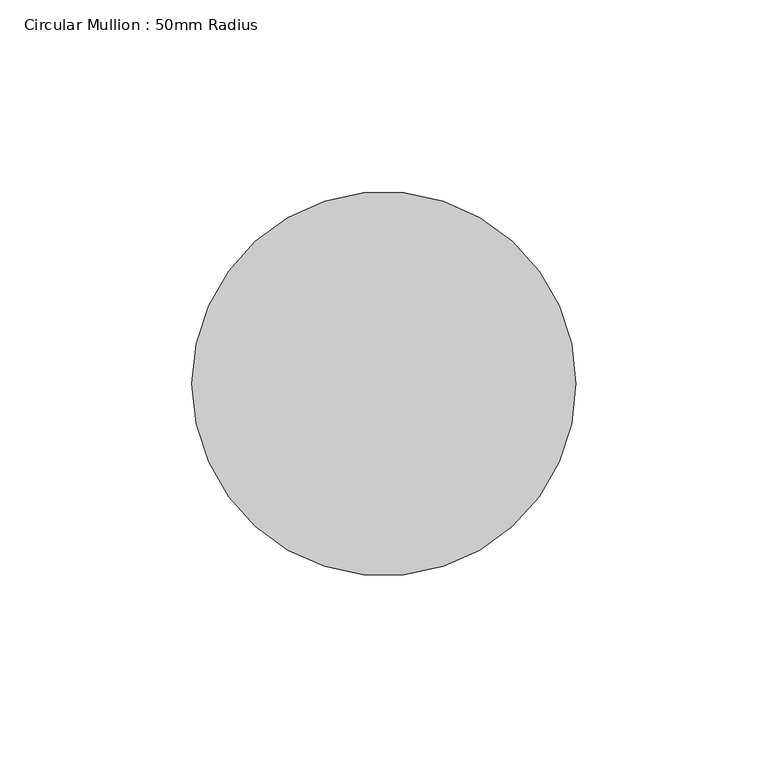
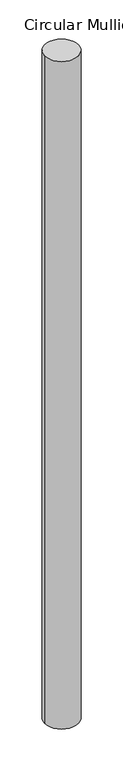
"""IFC4 building model written with IfcOpenShell, lengths in millimetres: member geometry, Circular Mullion : 50mm Radius."""

from ifc_helpers import new_model, si_unit, point, frame, frame_2d, origin, place, context, project, spatial, circle_curve, trimmed, segment, composite_curve, outline, extrude, source, transform, mapped, element, save


def circular_mullion_50mm_radius_f1cf2dd3(model_context):
    return source(origin(), model_context, "Body", "SweptSolid", [
        extrude(outline(composite_curve([segment(trimmed(circle_curve(frame_2d((-50.0, 0.0)), 50.0), [point((0.0, 0.0))], [point((-100.0, 0.0))], False, "CARTESIAN"), True, "CONTINUOUS"), segment(trimmed(circle_curve(frame_2d((-50.0, 0.0)), 50.0), [point((-100.0, 0.0))], [point((0.0, 0.0))], False, "CARTESIAN"), True, "CONTINUOUS")], self_intersect=False)), frame((0.0, 0.0, -2073.8472167), z_axis=(0.0, 0.0, 1.0), x_axis=(1.0, 0.0, 0.0)), (0.0, 0.0, 1.0), 2073.8472167),
    ])


if __name__ == "__main__":
    model = new_model("IFC4")
    model_context = context("Model", 3, world=origin())
    ifc_project = project(units=[si_unit("LENGTHUNIT", "METRE", prefix="MILLI")], contexts=[model_context])
    site = spatial("IfcSite", under=ifc_project)
    building = spatial("IfcBuilding", under=site)
    placement = place(None, origin())
    circular_mullion_50mm_radius_shape = circular_mullion_50mm_radius_f1cf2dd3(model_context)
    element("IfcMember", 1, ObjectType="Circular Mullion : 50mm Radius", at=placement, inside=building, context=model_context, shape_type="MappedRepresentation", body=[
        mapped(circular_mullion_50mm_radius_shape, transform((0.0, 0.0, 0.0), x_axis=(1.0, 0.0, 0.0), y_axis=(0.0, 1.0, 0.0), z_axis=(0.0, 0.0, 1.0))),
    ])
    save(model, "model.ifc")

# Revit data of these elements
# Type "Circular Mullion : 50mm Radius"
#   built-in parameter 1007350 = 0.164042 (stored number, unit not read)
# Element 1 (IfcMember, "Circular Mullion : 50mm Radius")
#   Materials on its faces: "Aluminium"
# Materials
#   "Aluminium": class "Metal", colour RGB 247 247 247, transparency 0, Description = "Aluminium 6061", Cost = 0
